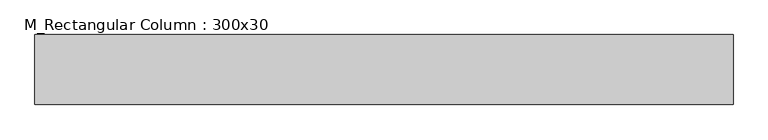
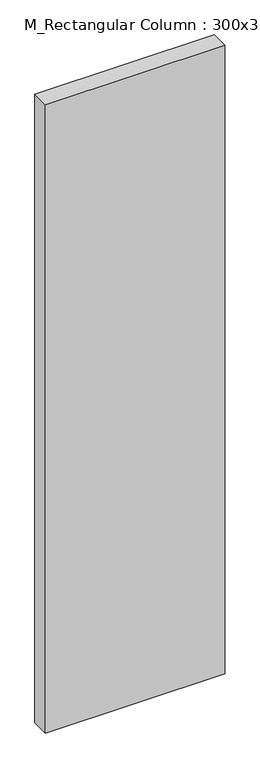
"""IFC4 building model written with IfcOpenShell, lengths in millimetres: column geometry, M_Rectangular Column : 300x30."""

from ifc_helpers import new_model, si_unit, frame, origin, place, context, project, spatial, polyline, outline, extrude, source, transform, mapped, element, save


def m_rectangular_column_300x30_baf48ca4(model_context):
    return source(origin(), model_context, "Body", "SweptSolid", [
        extrude(outline(polyline([(1500.0, -150.0), (-1500.0, -150.0), (-1500.0, 150.0), (1500.0, 150.0), (1500.0, -150.0)])), frame((0.0, 0.0, -3200.0), z_axis=(0.0, 0.0, 1.0), x_axis=(1.0, 0.0, 0.0)), (0.0, 0.0, 1.0), 11100.0),
    ])


if __name__ == "__main__":
    model = new_model("IFC4")
    model_context = context("Model", 3, world=origin())
    ifc_project = project(units=[si_unit("LENGTHUNIT", "METRE", prefix="MILLI")], contexts=[model_context])
    site = spatial("IfcSite", under=ifc_project)
    building = spatial("IfcBuilding", under=site)
    placement = place(None, origin())
    m_rectangular_column_300x30_shape = m_rectangular_column_300x30_baf48ca4(model_context)
    element("IfcColumn", 1, ObjectType="M_Rectangular Column : 300x30", at=placement, inside=building, context=model_context, shape_type="MappedRepresentation", body=[
        mapped(m_rectangular_column_300x30_shape, transform((0.0, 0.0, 0.0), x_axis=(1.0, 0.0, 0.0), y_axis=(0.0, 1.0, 0.0), z_axis=(0.0, 0.0, 1.0))),
    ])
    save(model, "model.ifc")

# Revit data of these elements
# Type "M_Rectangular Column : 300x30"
#   Depth = 30 cm
#   Offset Base = 0 cm
#   Offset Top = 0 cm
#   Width = 300 cm
#   Material = none
